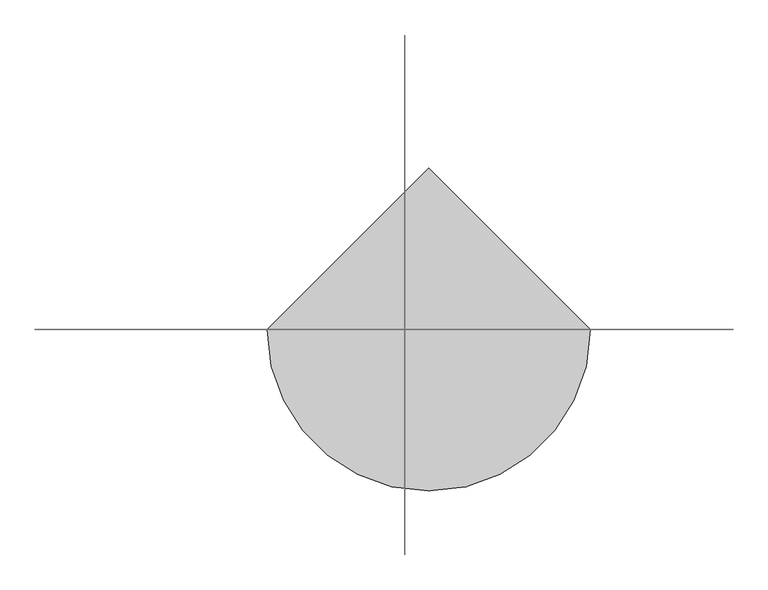
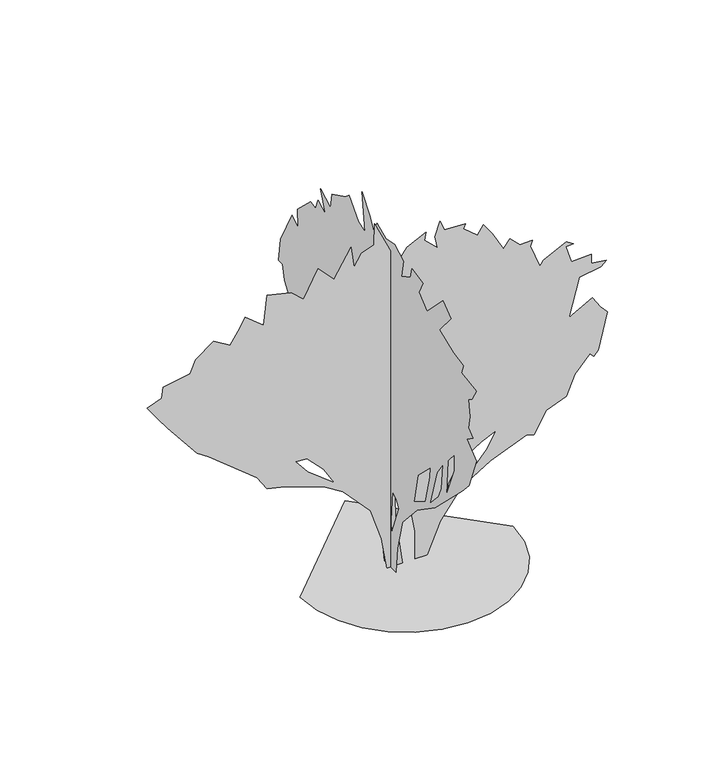
"""IFC4 building model written with IfcOpenShell, lengths in millimetres: proxy geometry, honey myrtle 26117 : honey myrtle 26117."""

import ifcopenshell
import ifcopenshell.guid

model = None  # the IFC model being written
_history = None  # IfcOwnerHistory: only IFC2X3 demands one
_inside = {}  # id of a spatial element -> (the spatial element, [elements in it])
_under = {}  # id of a project, library or spatial element -> (it, [spatial elements below it])
_declared = {}  # id of a project -> (the project, [libraries it declares])
_typed = {}  # id of a type object -> (the type object, [elements of that type])
_made_of = {}  # id of a material, layer set ... -> (it, [elements and type objects made of it])


def new_model(schema):
    """Start an empty IFC model of exactly this schema.

    Asked for "IFC4X3", IfcOpenShell would pick the latest addendum, in which some entities
    have other attributes; the version numbers below select the first issue.
    IFC2X3 requires an IfcOwnerHistory on every rooted entity: one is made here for all.
    """
    global model, _history
    if schema == "IFC4X3":
        model = ifcopenshell.file(schema_version=(4, 3, 0, 0))
    else:
        model = ifcopenshell.file(schema=schema)
    _inside.clear()
    _under.clear()
    _declared.clear()
    _typed.clear()
    _made_of.clear()
    _history = None
    if model.schema == "IFC2X3":
        org = make("IfcOrganization", Name="unknown")
        user = make(
            "IfcPersonAndOrganization",
            ThePerson=make("IfcPerson", FamilyName="unknown"),
            TheOrganization=org,
        )
        app = make(
            "IfcApplication",
            ApplicationDeveloper=org,
            Version="unknown",
            ApplicationFullName="unknown",
            ApplicationIdentifier="unknown",
        )
        _history = make(
            "IfcOwnerHistory",
            OwningUser=user,
            OwningApplication=app,
            ChangeAction="ADDED",
            CreationDate=0,
        )
    return model


def make(cls, **values):
    """One entity of the class cls with the attributes given. An attribute that is None is left unset."""
    return model.create_entity(
        cls, **{name: value for name, value in values.items() if value is not None}
    )


def rooted(cls, **values):
    """An entity with a GlobalId (a new one), such as an element, a storey or a relation."""
    return make(cls, GlobalId=ifcopenshell.guid.new(), OwnerHistory=_history, **values)


def si_unit(unit_type, name, prefix=None):
    """IfcSIUnit, for example si_unit("LENGTHUNIT", "METRE", prefix="MILLI")."""
    return make("IfcSIUnit", UnitType=unit_type, Prefix=prefix, Name=name)


def assignment(units):
    """IfcUnitAssignment: the units of a project."""
    return None if units is None else make("IfcUnitAssignment", Units=units)


def point(xyz):
    """IfcCartesianPoint."""
    return None if xyz is None else make("IfcCartesianPoint", Coordinates=xyz)


def direction(xyz):
    """IfcDirection."""
    return None if xyz is None else make("IfcDirection", DirectionRatios=xyz)


def frame(location, z_axis=None, x_axis=None):
    """IfcAxis2Placement3D, a coordinate frame: its origin and axes. An axis left out is left unset."""
    return make(
        "IfcAxis2Placement3D",
        Location=point(location),
        Axis=direction(z_axis),
        RefDirection=direction(x_axis),
    )


def origin():
    """The frame at (0, 0, 0) with its axes left unset."""
    return frame((0.0, 0.0, 0.0))


def place(relative_to, where):
    """IfcLocalPlacement: puts the frame where relative to a parent placement (None: the world)."""
    return make(
        "IfcLocalPlacement", PlacementRelTo=relative_to, RelativePlacement=where
    )


def context(
    kind, dimensions, precision=None, world=None, true_north=None, identifier=None
):
    """IfcGeometricRepresentationContext, for example the 3D "Model" context."""
    return make(
        "IfcGeometricRepresentationContext",
        ContextIdentifier=identifier,
        ContextType=kind,
        CoordinateSpaceDimension=dimensions,
        Precision=precision,
        WorldCoordinateSystem=world,
        TrueNorth=true_north,
    )


def project(units=None, contexts=None):
    """IfcProject with its units and contexts."""
    return rooted(
        "IfcProject",
        Name="project",
        RepresentationContexts=contexts,
        UnitsInContext=assignment(units),
    )


def spatial(cls, under=None, at=None, **own):
    """A site, building, storey or space (cls), placed at a placement, below another one or the project."""
    s = rooted(cls, ObjectPlacement=at, **own)
    if under is not None:
        _under.setdefault(under.id(), (under, []))[1].append(s)
    return s


def point_list(points):
    """IfcCartesianPointList2D or 3D."""
    cls = (
        "IfcCartesianPointList2D" if len(points[0]) == 2 else "IfcCartesianPointList3D"
    )
    return make(cls, CoordList=points)


def triangles(points, corners, closed=None, point_numbers=None):
    """IfcTriangulatedFaceSet: each triangle names its three corners, points numbered from 1."""
    return make(
        "IfcTriangulatedFaceSet",
        Coordinates=point_list(points),
        Closed=closed,
        CoordIndex=corners,
        PnIndex=point_numbers,
    )


def shape(context_of_items, identifier, shape_type, items):
    """IfcShapeRepresentation: the items that make up one representation, for example the "Body"."""
    return make(
        "IfcShapeRepresentation",
        ContextOfItems=context_of_items,
        RepresentationIdentifier=identifier,
        RepresentationType=shape_type,
        Items=items,
    )


def source(mapping_origin, context_of_items, identifier, shape_type, items):
    """IfcRepresentationMap: a shape defined once, which mapped items show again and again."""
    return make(
        "IfcRepresentationMap",
        MappingOrigin=mapping_origin,
        MappedRepresentation=shape(context_of_items, identifier, shape_type, items),
    )


def transform(
    local_origin,
    x_axis=None,
    y_axis=None,
    z_axis=None,
    scale=None,
    scale2=None,
    scale3=None,
    uniform=True,
):
    """IfcCartesianTransformationOperator3D, or its non-uniform kind. x_axis, y_axis, z_axis: its Axis1, 2, 3."""
    if uniform:
        return make(
            "IfcCartesianTransformationOperator3D",
            Axis1=direction(x_axis),
            Axis2=direction(y_axis),
            LocalOrigin=point(local_origin),
            Scale=scale,
            Axis3=direction(z_axis),
        )
    return make(
        "IfcCartesianTransformationOperator3DnonUniform",
        Axis1=direction(x_axis),
        Axis2=direction(y_axis),
        LocalOrigin=point(local_origin),
        Scale=scale,
        Axis3=direction(z_axis),
        Scale2=scale2,
        Scale3=scale3,
    )


def mapped(mapping_source, mapping_target):
    """IfcMappedItem: shows the shape of a source again, moved by a transform."""
    return make(
        "IfcMappedItem", MappingSource=mapping_source, MappingTarget=mapping_target
    )


def made_of(thing, what):
    """Note that an element or type object is made of a material, layer set ...; save() writes the relation."""
    if what is not None:
        _made_of.setdefault(what.id(), (what, []))[1].append(thing)
    return thing


def element(
    cls,
    number,
    at=None,
    inside=None,
    cuts=None,
    type_object=None,
    material=None,
    context=None,
    identifier="Body",
    shape_type=None,
    held_by="IfcProductDefinitionShape",
    body=None,
    shapes=None,
    **own,
):
    """One element of the class cls, such as IfcWall. Its Tag is "e" and its number.

    at: its placement. inside: the storey or other place that contains it. cuts: it is an
    opening in that element (IfcRelVoidsElement). A single representation is given by context,
    identifier, shape_type and body (its items); several are given by shapes. held_by: the class
    of the entity that holds the representations. save() writes the other relations.
    """
    e = rooted(cls, Tag="e%d" % number, ObjectPlacement=at, **own)
    if body is not None:
        shapes = [shape(context, identifier, shape_type, body)]
    if shapes is not None:
        e.Representation = make(held_by, Representations=shapes)
    if inside is not None:
        _inside.setdefault(inside.id(), (inside, []))[1].append(e)
    if cuts is not None:
        rooted(
            "IfcRelVoidsElement", RelatingBuildingElement=cuts, RelatedOpeningElement=e
        )
    if type_object is not None:
        _typed.setdefault(type_object.id(), (type_object, []))[1].append(e)
    return made_of(e, material)


def aggregate(whole, parts):
    """IfcRelAggregates: a whole, such as a stair, and the parts it consists of."""
    return rooted("IfcRelAggregates", RelatingObject=whole, RelatedObjects=parts)


def save(model, path):
    """Write the relations noted so far, then the file.

    IfcRelAggregates (storeys below a building ...), IfcRelContainedInSpatialStructure (elements
    in a storey), IfcRelDefinesByType, IfcRelAssociatesMaterial and IfcRelDeclares: one each for
    every whole, place, type object, material and project.
    """
    for whole, parts in _under.values():
        aggregate(whole, parts)
    for where, things in _inside.values():
        rooted(
            "IfcRelContainedInSpatialStructure",
            RelatedElements=things,
            RelatingStructure=where,
        )
    for kind, things in _typed.values():
        rooted("IfcRelDefinesByType", RelatedObjects=things, RelatingType=kind)
    for what, things in _made_of.values():
        rooted("IfcRelAssociatesMaterial", RelatedObjects=things, RelatingMaterial=what)
    for by, libraries in _declared.values():
        rooted("IfcRelDeclares", RelatingContext=by, RelatedDefinitions=libraries)
    model.write(path)


def entourage_6475341c(model_context):
    return source(origin(), model_context, "Body", "Tessellation", [
        triangles([(-396.3767504, 0.0, 8.22e-05), (-385.8992649, -90.8237077, 8.22e-05), (-356.0543206, -174.2306261, 8.22e-05), (-309.2370838, -247.8313661, 8.22e-05), (-247.8313661, -309.2370838, 8.22e-05), (-174.2306261, -356.0543206, 8.22e-05), (-90.8237077, -385.8992649, 8.22e-05), (1.73e-05, -396.3767504, 8.22e-05), (90.8237077, -385.8992649, 8.22e-05), (174.2306261, -356.0543206, 8.22e-05), (247.8313661, -309.2370838, 8.22e-05), (309.2370838, -247.8313661, 8.22e-05), (356.0543206, -174.2306261, 8.22e-05), (385.8992649, -90.8237077, 8.22e-05), (396.3767504, 3.47e-05, 8.22e-05), (-5.2e-05, 396.3767504, 8.22e-05), (-59.3577095, -35.0059915, 9.26e-05), (-59.3577095, -44.8705806, 101.5460546), (-59.3577095, -75.4742449, 222.0478563), (-59.3577095, -168.9964434, 326.3007588), (-59.3577095, -285.8741748, 405.6706235), (-59.3579639, -459.2340692, 576.3228888), (-59.3579639, -503.9253456, 625.6344137), (-59.3579639, -553.1479589, 751.1941189), (-59.3579639, -491.6190474, 799.7715317), (-59.3579639, -530.478485, 828.915465), (-59.3579639, -501.3320083, 851.5849388), (-59.3579639, -511.0474763, 900.1598808), (-59.3579639, -501.3320083, 961.688756), (-59.3579639, -524.0014821, 977.8812269), (-59.3579639, -553.1479589, 1026.4561689), (-59.3579639, -455.9955677, 1039.4101748), (-59.3579639, -469.4956884, 1077.0376745), (-59.3579639, -404.1821606, 1087.9850441), (-59.3579639, -313.5068087, 1123.6085238), (-59.3579639, -387.9896896, 1211.0454105), (-59.3579639, -336.1762825, 1249.9048119), (-59.3579639, -235.7859349, 1149.5164627), (-59.3579639, -183.9712561, 1191.6144018), (-59.3579639, -209.8784683, 1243.4278816), (-59.3579639, -138.9198272, 1256.3183739), (-59.3579639, -128.9188388, 1217.5224134), (-59.3579639, -70.6279291, 1185.1373989), (-59.3579639, -83.5816624, 1253.143277), (-59.3579639, -25.4436618, 1284.1769932), (-59.3579639, 29.761912, 1272.5743584), (-59.3579639, 86.0073592, 1299.3586246), (-59.3579639, 110.7212849, 1256.3817421), (-59.3579639, 133.3899957, 1298.4822247), (-59.3579639, 185.2039207, 1363.2496376), (-59.3577095, 165.7739475, 1217.5224134), (-59.3577095, 207.8728858, 1230.4738758), (-59.3577095, 266.3644464, 1299.9199276), (-59.3577095, 292.0717617, 1279.0512886), (-59.3577095, 376.2676217, 1236.950806), (-59.3577095, 385.9830897, 1178.660396), (-59.3577095, 450.7505027, 1214.2838757), (-59.3577095, 418.3680679, 1133.3239918), (-59.3577095, 466.9429736, 1159.22946), (-59.3577095, 484.2835213, 1117.1086298), (-59.3577095, 515.5204227, 1123.6085238), (-59.3577095, 599.7162646, 1042.6486399), (-59.3577095, 596.4777632, 974.6427618), (-59.3577095, 635.3397079, 997.3122356), (-59.3577095, 709.8225889, 858.0619417), (-59.3577095, 722.7765947, 767.3865898), (-59.3577095, 696.8686558, 767.3865898), (-59.3577095, 683.91465, 712.3346449), (-59.3577095, 619.147237, 621.659293), (-59.3577095, 586.7622588, 628.1362959), (-59.3577095, 577.0493342, 595.7513177), (-59.3577095, 544.664356, 589.2743148), (-59.3577095, 512.2819213, 514.7914338), (-59.3577095, 453.9890041, 501.8400078), (-59.3577095, 473.4199765, 479.1705339), (-59.3577095, 438.083507, 433.2245012), (-59.3577095, 424.8450708, 430.5955919), (-59.3577095, 359.671251, 388.3935531), (-59.3577095, 230.5626891, 332.9860339), (-59.3577095, 112.6590482, 224.7923109), (-59.3577095, 55.1474106, 87.2636415), (-59.3577095, 39.476642, 8.38e-05), (-59.3577095, -5.8605105, 135.9018064), (-59.3577095, -2.7896791, 186.1833303), (-59.3577095, -12.337225, 304.2967785), (-59.3577095, -38.2442317, 288.1068329), (-59.3577095, -54.4362076, 262.1988576), (-59.3577095, -151.5875587, 349.6357444), (-59.3577095, -177.4947618, 469.4550296), (-59.3577095, -258.4549001, 547.176412), (-59.3577095, -255.2163986, 508.3169744), (-59.3577095, -226.0704487, 394.9721486), (-59.3577095, -255.2163986, 404.687653), (-59.3577095, -297.3143196, 550.4149135), (-59.3577095, -337.517407, 606.5056758), (-59.3577095, -326.4607781, 505.0785092), (-59.3577095, -307.0298058, 462.9780267), (-59.3577095, -358.8432129, 501.8400078), (-59.3579639, -368.5587173, 641.0903017), (-59.3579639, -410.6591635, 689.6651711), (-59.3579639, -410.6591635, 628.1362959), (-59.3577095, 198.157654, 356.112711), (-59.3577095, 261.769596, 391.7057055), (-59.3577095, 324.4541782, 475.9320325), (-59.3577095, 282.3562755, 469.4550296), (-59.3577095, 253.2100531, 430.5955919), (-267.2940953, 2.61e-05, 404.687653), (-308.6096875, 2.21e-05, 471.3142911), (-370.9208914, 1.84e-05, 534.2224425), (-413.0213739, 1.82e-05, 537.4609076), (-368.4215527, 2.15e-05, 482.1804156), (30.6369404, 5.02e-05, 0.0), (31.1304627, 4.38e-05, 108.1619844), (9.0696959, 3.61e-05, 237.4841779), (-47.0839311, 3.05e-05, 330.2047357), (-39.4309189, 4.01e-05, 170.4041154), (-14.7000316, 5.02e-05, 0.0), (-72.990889, 5.02e-05, 0.0), (-92.9872747, 4.29e-05, 122.5858678), (-134.4006626, 3.55e-05, 247.1552083), (-236.0793036, 2.88e-05, 358.7517941), (-302.2063538, 2.64e-05, 398.8659516), (-451.8807753, 2.32e-05, 453.2625587), (-519.8892331, 2.22e-05, 469.4550296), (-555.510133, 1.89e-05, 524.5069382), (-736.858366, 1.03e-05, 670.234235), (-778.9587759, 8.5e-06, 699.3807117), (-889.0625931, 4e-07, 835.3924679), (-924.6860727, -2.5e-06, 883.9674099), (-965.6003632, -6e-06, 942.4685629), (-911.7320669, -7.1e-06, 961.688756), (-905.255064, -9.6e-06, 1003.7892385), (-804.8642441, -1.06e-05, 1019.979166), (-785.4357788, -1.35e-05, 1068.5565788), (-717.4299007, -1.64e-05, 1117.1315208), (-655.8984821, -1.43e-05, 1081.5105846), (-620.2775459, -1.75e-05, 1136.5625296), (-600.8465735, -1.97e-05, 1172.1833931), (-532.8406591, -1.64e-05, 1117.1315208), (-519.8892331, -2.31e-05, 1230.4738758), (-429.2138449, -2.18e-05, 1207.8068727), (-383.8748972, -1.93e-05, 1165.7064629), (-328.8229886, -2.53e-05, 1266.0972828), (-270.5325967, -2.16e-05, 1204.5684076), (-205.7644389, -2.78e-05, 1308.1951492), (-196.0496976, -2.29e-05, 1227.2378815), (-167.6639666, -2.55e-05, 1270.8241745), (-121.5665623, -2.66e-05, 1288.7668293), (-119.7654549, -3.15e-05, 1371.5986919), (-34.1304544, -2.06e-05, 1188.3759367), (2.3015577, -2.34e-05, 1235.4267712), (72.7363851, -2.54e-05, 1269.3357479), (66.2596456, -2.37e-05, 1240.1892712), (114.8353143, -2.1e-05, 1194.8529396), (105.1200825, -2.37e-05, 1240.1892712), (124.5505553, -2.7e-05, 1295.2437595), (140.7425266, -2.47e-05, 1256.3817421), (218.4636638, -2.45e-05, 1253.143277), (211.1367854, -2.35e-05, 1235.7950626), (263.8015941, -2.08e-05, 1191.6144018), (286.4685245, -2.27e-05, 1223.9994164), (318.8535027, -2e-05, 1178.660396), (360.9514054, -1.56e-05, 1104.177515), (385.0814006, -1.75e-05, 1135.7446289), (422.4828604, -1.52e-05, 1097.7005121), (467.8192646, -1.54e-05, 1100.9390499), (461.3422617, -1.41e-05, 1078.2721195), (496.9657413, -8.7e-06, 987.5967676), (509.9172037, -9.8e-06, 1007.0277037), (594.1155527, -1.23e-05, 1049.1256428), (620.0235643, -1.14e-05, 1032.9331718), (593.290058, -1.13e-05, 1031.1069025), (613.5465614, -7.3e-06, 964.9272211), (688.0294424, -7.5e-06, 968.1657589), (688.0294424, -5.4e-06, 932.5448227), (743.0813147, -5e-06, 926.0678198), (723.6503786, -3.8e-06, 906.6368837), (642.6904947, -3.1e-06, 893.6828779), (603.8310571, 5.6e-06, 747.9555811), (691.2679075, 2.7e-06, 796.5330666), (720.4118408, 5.4e-06, 751.1941189), (746.3198524, 7.2e-06, 722.0501856), (713.9348379, 1.55e-05, 582.7973482), (697.7449104, 1.66e-05, 563.3688829), (681.5524395, 1.57e-05, 579.5613902), (626.5005672, 1.93e-05, 518.0299353), (594.1155527, 2.38e-05, 443.5470543), (519.6326717, 2.55e-05, 414.403121), (474.2962675, 3.03e-05, 333.4432371), (448.3882922, 2.98e-05, 343.1587415), (311.7719945, 3.3e-05, 288.0331637), (205.1723602, 3.7e-05, 221.2502851), (125.3034072, 4.32e-05, 117.1220752), (75.9746277, 5.02e-05, 0.0), (30.6369404, 3.34e-05, 281.62983), (43.5909303, 2.72e-05, 385.2566442), (7.9686832, 2.28e-05, 459.7395252), (-30.8919575, 2.45e-05, 430.5955919), (-38.6976243, 2.72e-05, 386.112624), (-2.6646859, 3.14e-05, 315.8842435), (150.4575132, 3.75e-05, 213.6229345), (215.0437962, 3.57e-05, 242.9182394), (296.5269221, 3.01e-05, 337.5199505), (331.8074721, 2.65e-05, 398.2106501), (278.0814637, 2.79e-05, 375.0661689), (195.3344433, 3.11e-05, 320.3901821), (154.7673882, 3.52e-05, 251.8887493)], [[15, 16, 1], [14, 15, 1], [14, 1, 2], [13, 14, 2], [13, 2, 3], [13, 3, 4], [12, 13, 4], [11, 12, 4], [11, 4, 5], [11, 5, 6], [11, 6, 7], [11, 7, 8], [11, 8, 9], [11, 9, 10], [93, 90, 91], [93, 91, 92], [90, 93, 94], [95, 98, 99], [83, 17, 18], [98, 95, 96], [49, 50, 51], [56, 57, 58], [88, 85, 86], [48, 49, 51], [102, 84, 85], [83, 18, 19], [87, 83, 19], [30, 31, 32], [87, 19, 20], [39, 40, 41], [39, 41, 42], [25, 26, 27], [29, 30, 32], [82, 17, 83], [81, 82, 83], [80, 81, 83], [80, 83, 84], [80, 84, 102], [79, 80, 102], [79, 102, 103], [78, 79, 103], [78, 103, 104], [77, 78, 104], [32, 33, 34], [65, 66, 67], [58, 59, 60], [35, 36, 37], [35, 37, 38], [88, 86, 87], [88, 87, 20], [92, 88, 20], [92, 20, 21], [93, 92, 21], [97, 93, 21], [97, 21, 22], [63, 64, 65], [52, 53, 54], [46, 47, 48], [74, 75, 76], [23, 24, 25], [43, 44, 45], [43, 45, 46], [98, 96, 97], [98, 97, 22], [101, 98, 22], [101, 22, 23], [101, 23, 25], [100, 101, 25], [68, 69, 70], [74, 76, 77], [74, 77, 104], [70, 71, 72], [85, 88, 89], [102, 85, 89], [106, 102, 89], [105, 106, 89], [52, 54, 55], [52, 55, 56], [60, 61, 62], [60, 62, 63], [39, 42, 43], [72, 73, 74], [43, 46, 48], [43, 48, 51], [63, 65, 67], [90, 94, 95], [105, 89, 90], [38, 39, 43], [63, 67, 68], [63, 68, 70], [63, 70, 72], [60, 63, 72], [58, 60, 72], [58, 72, 74], [58, 74, 104], [58, 104, 105], [58, 105, 90], [56, 58, 90], [52, 56, 90], [51, 52, 90], [43, 51, 90], [38, 43, 90], [38, 90, 95], [38, 95, 99], [38, 99, 100], [35, 38, 100], [35, 100, 25], [35, 25, 27], [34, 35, 27], [32, 34, 27], [29, 32, 27], [28, 29, 27], [196, 112, 113], [196, 197, 201], [195, 196, 113], [195, 113, 114], [148, 149, 150], [112, 196, 201], [170, 171, 172], [207, 201, 197], [144, 145, 146], [155, 156, 157], [175, 176, 177], [175, 177, 178], [151, 152, 153], [194, 112, 201], [193, 194, 201], [192, 193, 201], [192, 201, 202], [191, 192, 202], [191, 202, 203], [195, 114, 115], [200, 195, 115], [199, 200, 115], [169, 170, 172], [206, 207, 197], [157, 158, 159], [165, 166, 167], [160, 161, 162], [142, 143, 144], [129, 130, 131], [116, 117, 118], [116, 118, 119], [116, 119, 120], [115, 116, 120], [107, 115, 120], [107, 120, 121], [107, 121, 122], [111, 107, 122], [111, 122, 123], [110, 111, 123], [137, 138, 139], [199, 115, 107], [163, 164, 165], [139, 140, 141], [183, 184, 185], [190, 191, 203], [190, 203, 204], [173, 174, 175], [173, 175, 178], [169, 172, 173], [179, 180, 181], [198, 199, 107], [139, 141, 142], [188, 189, 190], [110, 123, 124], [110, 124, 125], [168, 169, 173], [154, 155, 157], [154, 157, 159], [131, 132, 133], [182, 183, 185], [188, 190, 204], [147, 148, 150], [146, 147, 150], [205, 206, 197], [136, 137, 139], [181, 182, 185], [179, 181, 185], [179, 185, 186], [134, 135, 136], [198, 107, 108], [154, 159, 160], [133, 134, 136], [168, 173, 178], [168, 178, 179], [129, 131, 133], [128, 129, 133], [127, 128, 133], [127, 133, 136], [126, 127, 136], [126, 136, 139], [125, 126, 139], [110, 125, 139], [110, 139, 142], [109, 110, 142], [109, 142, 144], [109, 144, 146], [109, 146, 150], [108, 109, 150], [198, 108, 150], [197, 198, 150], [205, 197, 150], [204, 205, 150], [188, 204, 150], [187, 188, 150], [186, 187, 150], [179, 186, 150], [168, 179, 150], [167, 168, 150], [150, 151, 153], [150, 153, 154], [160, 162, 163], [154, 160, 163], [150, 154, 163], [167, 150, 163], [167, 163, 165]], closed=False),
    ])


if __name__ == "__main__":
    model = new_model("IFC4")
    model_context = context("Model", 3, world=origin())
    ifc_project = project(units=[si_unit("LENGTHUNIT", "METRE", prefix="MILLI")], contexts=[model_context])
    site = spatial("IfcSite", under=ifc_project)
    building = spatial("IfcBuilding", under=site)
    placement = place(None, origin())
    entourage_shape = entourage_6475341c(model_context)
    element("IfcBuildingElementProxy", 1, Name="honey myrtle 26117 : honey myrtle 26117", ObjectType="honey myrtle 26117 : honey myrtle 26117", at=placement, inside=building, context=model_context, shape_type="MappedRepresentation", body=[
        mapped(entourage_shape, transform((0.0, 0.0, 0.0), x_axis=(1.0, 0.0, 0.0), y_axis=(0.0, 1.0, 0.0), z_axis=(0.0, 0.0, 1.0))),
    ])
    save(model, "model.ifc")

# Revit data of these elements
# Type "honey myrtle 26117 : honey myrtle 26117"
#   built-in parameter 1005195 = "RPC-16-G3GK-N2Q0-PN0G-6000-ST1L-LVER-AU"
#   Height = 0
